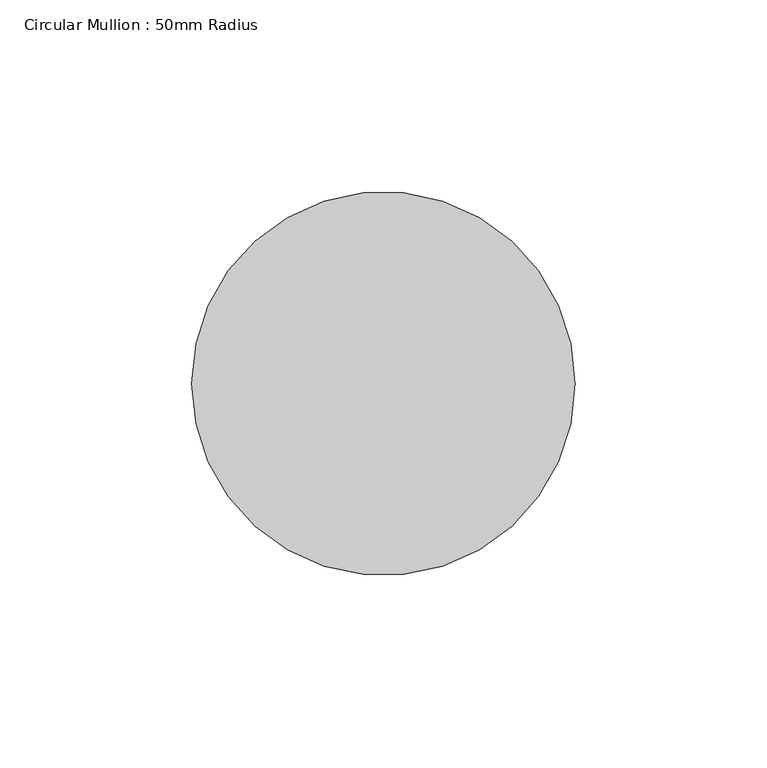
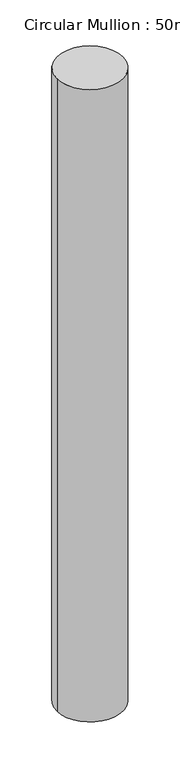
"""IFC4 building model written with IfcOpenShell, lengths in millimetres: member geometry, Circular Mullion : 50mm Radius."""

from ifc_helpers import new_model, si_unit, point, frame, origin, origin_2d, place, context, project, spatial, circle_curve, trimmed, segment, composite_curve, outline, extrude, source, transform, mapped, element, save


def circular_mullion_50mm_radius_064a8777(model_context):
    return source(origin(), model_context, "Body", "SweptSolid", [
        extrude(outline(composite_curve([segment(trimmed(circle_curve(origin_2d(), 50.0), [point((50.0, 0.0))], [point((-50.0, 0.0))], False, "CARTESIAN"), True, "CONTINUOUS"), segment(trimmed(circle_curve(origin_2d(), 50.0), [point((-50.0, 0.0))], [point((50.0, 0.0))], False, "CARTESIAN"), True, "CONTINUOUS")], self_intersect=False)), frame((0.0, 0.0, -1015.7355903), z_axis=(0.0, 0.0, 1.0), x_axis=(1.0, 0.0, 0.0)), (0.0, 0.0, 1.0), 1015.7355903),
    ])


if __name__ == "__main__":
    model = new_model("IFC4")
    model_context = context("Model", 3, world=origin())
    ifc_project = project(units=[si_unit("LENGTHUNIT", "METRE", prefix="MILLI")], contexts=[model_context])
    site = spatial("IfcSite", under=ifc_project)
    building = spatial("IfcBuilding", under=site)
    placement = place(None, origin())
    circular_mullion_50mm_radius_shape = circular_mullion_50mm_radius_064a8777(model_context)
    element("IfcMember", 1, ObjectType="Circular Mullion : 50mm Radius", at=placement, inside=building, context=model_context, shape_type="MappedRepresentation", body=[
        mapped(circular_mullion_50mm_radius_shape, transform((0.0, 0.0, 0.0), x_axis=(1.0, 0.0, 0.0), y_axis=(0.0, 1.0, 0.0), z_axis=(0.0, 0.0, 1.0))),
    ])
    save(model, "model.ifc")

# Revit data of these elements
# Type "Circular Mullion : 50mm Radius"
#   built-in parameter 1007350 = 0.164042 (stored number, unit not read)
# Element 1 (IfcMember, "Circular Mullion : 50mm Radius")
#   Materials on its faces: "Aluminium"
# Materials
#   "Aluminium": class "Metal", colour RGB 247 247 247, transparency 0, Description = "Aluminium 6061", Cost = 0
